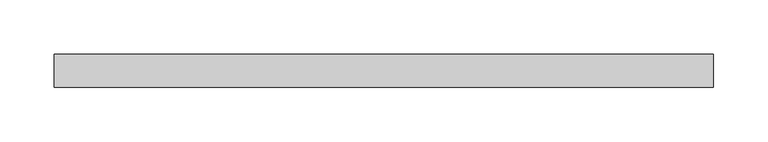
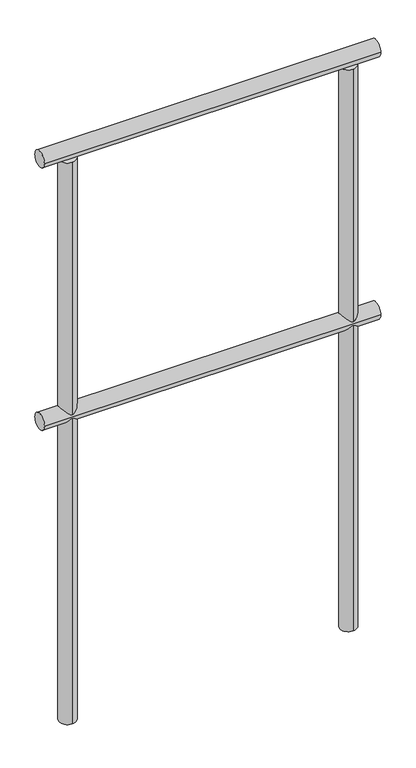
"""IFC4 building model written with IfcOpenShell, lengths in millimetres: railing geometry."""

from ifc_helpers import new_model, si_unit, point, frame, frame_2d, origin, place, context, project, spatial, circle_curve, trimmed, segment, composite_curve, outline, extrude, source, transform, mapped, element, save


def railing_c3f589da(model_context):
    return source(origin(), model_context, "Body", "SweptSolid", [
        extrude(outline(composite_curve([segment(trimmed(circle_curve(frame_2d((33021.2934796, 885.0)), 15.0), [point((33036.2934796, 885.0))], [point((33006.2934796, 885.0))], False, "CARTESIAN"), True, "CONTINUOUS"), segment(trimmed(circle_curve(frame_2d((33021.2934796, 885.0)), 15.0), [point((33006.2934796, 885.0))], [point((33036.2934796, 885.0))], False, "CARTESIAN"), True, "CONTINUOUS")], self_intersect=False)), frame((-1056.0, 0.0, 0.0), z_axis=(1.0, 0.0, 0.0), x_axis=(0.0, 1.0, 0.0)), (0.0, 0.0, 1.0), 606.0),
        extrude(outline(composite_curve([segment(trimmed(circle_curve(frame_2d((33021.2934796, 1385.0)), 15.0), [point((33036.2934796, 1385.0))], [point((33006.2934796, 1385.0))], False, "CARTESIAN"), True, "CONTINUOUS"), segment(trimmed(circle_curve(frame_2d((33021.2934796, 1385.0)), 15.0), [point((33006.2934796, 1385.0))], [point((33036.2934796, 1385.0))], False, "CARTESIAN"), True, "CONTINUOUS")], self_intersect=False)), frame((-1056.0, 0.0, 0.0), z_axis=(1.0, 0.0, 0.0), x_axis=(0.0, 1.0, 0.0)), (0.0, 0.0, 1.0), 606.0),
        extrude(outline(composite_curve([segment(trimmed(circle_curve(frame_2d((-1006.0, 33021.2934796)), 15.0), [point((-1006.0, 33036.2934796))], [point((-1006.0, 33006.2934796))], False, "CARTESIAN"), True, "CONTINUOUS"), segment(trimmed(circle_curve(frame_2d((-1006.0, 33021.2934796)), 15.0), [point((-1006.0, 33006.2934796))], [point((-1006.0, 33036.2934796))], False, "CARTESIAN"), True, "CONTINUOUS")], self_intersect=False)), frame((0.0, 0.0, 300.0), z_axis=(0.0, 0.0, 1.0), x_axis=(1.0, 0.0, 0.0)), (0.0, 0.0, 1.0), 1070.0),
        extrude(outline(composite_curve([segment(trimmed(circle_curve(frame_2d((-500.0, 33021.2934796)), 15.0), [point((-500.0, 33036.2934796))], [point((-500.0, 33006.2934796))], False, "CARTESIAN"), True, "CONTINUOUS"), segment(trimmed(circle_curve(frame_2d((-500.0, 33021.2934796)), 15.0), [point((-500.0, 33006.2934796))], [point((-500.0, 33036.2934796))], False, "CARTESIAN"), True, "CONTINUOUS")], self_intersect=False)), frame((0.0, 0.0, 300.0), z_axis=(0.0, 0.0, 1.0), x_axis=(1.0, 0.0, 0.0)), (0.0, 0.0, 1.0), 1070.0),
    ])


if __name__ == "__main__":
    model = new_model("IFC4")
    model_context = context("Model", 3, world=origin())
    ifc_project = project(units=[si_unit("LENGTHUNIT", "METRE", prefix="MILLI")], contexts=[model_context])
    site = spatial("IfcSite", under=ifc_project)
    building = spatial("IfcBuilding", under=site)
    placement = place(None, origin())
    railing_shape = railing_c3f589da(model_context)
    element("IfcRailing", 1, at=placement, inside=building, context=model_context, shape_type="MappedRepresentation", body=[
        mapped(railing_shape, transform((0.0, 0.0, 0.0), x_axis=(1.0, 0.0, 0.0), y_axis=(0.0, 1.0, 0.0), z_axis=(0.0, 0.0, 1.0))),
    ])
    save(model, "model.ifc")
